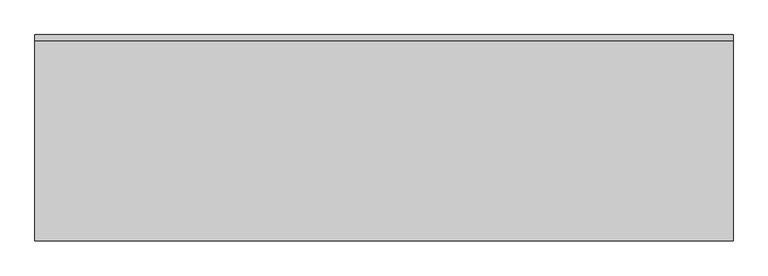
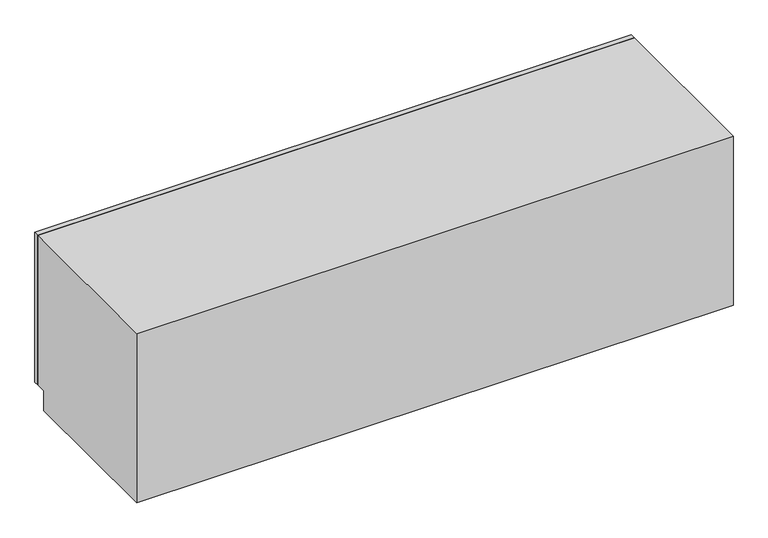
"""IFC4 building model written with IfcOpenShell, lengths in millimetres: furniture geometry, OD_CW_Base Cabinet : OD_CW_Base Cabinet."""

from ifc_helpers import new_model, si_unit, frame, origin, place, context, project, spatial, polyline, outline, extrude, source, transform, mapped, element, save


def furniture_ad26cfb4(model_context):
    return source(origin(), model_context, "Body", "SweptSolid", [
        extrude(outline(polyline([(18.7377049, 228.6), (18.7377049, 254.0), (2939.7377049, 254.0), (2939.7377049, 228.6), (18.7377049, 228.6)])), frame((0.0, 0.0, 101.6), z_axis=(0.0, 0.0, 1.0), x_axis=(1.0, 0.0, 0.0)), (0.0, 0.0, 1.0), 774.7),
        extrude(outline(polyline([(228.6, 876.3), (228.6, 101.6), (177.8, 101.6), (177.8, 0.0), (-609.6, 0.0), (-609.6, 876.3), (228.6, 876.3)])), frame((18.7377049, 0.0, 0.0), z_axis=(1.0, 0.0, 0.0), x_axis=(0.0, 1.0, 0.0)), (0.0, 0.0, 1.0), 2921.0),
    ])


if __name__ == "__main__":
    model = new_model("IFC4")
    model_context = context("Model", 3, world=origin())
    ifc_project = project(units=[si_unit("LENGTHUNIT", "METRE", prefix="MILLI")], contexts=[model_context])
    site = spatial("IfcSite", under=ifc_project)
    building = spatial("IfcBuilding", under=site)
    placement = place(None, origin())
    furniture_shape = furniture_ad26cfb4(model_context)
    element("IfcFurniture", 1, ObjectType="OD_CW_Base Cabinet : OD_CW_Base Cabinet", at=placement, inside=building, context=model_context, shape_type="MappedRepresentation", body=[
        mapped(furniture_shape, transform((0.0, 0.0, 0.0), x_axis=(1.0, 0.0, 0.0), y_axis=(0.0, 1.0, 0.0), z_axis=(0.0, 0.0, 1.0))),
    ])
    save(model, "model.ifc")

# Revit data of these elements
# Type "OD_CW_Base Cabinet : OD_CW_Base Cabinet"
#   OD_CW_Width [instance default] = 2' - 10"
#   OD_CW_Length [instance default] = 8' - 0"
#   OD_CW_Height [instance default] = 2' - 3"
#   Depth = 2' - 0"
#   Height = 3' - 0"
#   Width = 4' - 0"
#   OD_CW_Material_Front Panel [instance default] = none
#   OD_CW_Material_Body [instance default] = none
# Element 1 (IfcFurniture, "OD_CW_Base Cabinet : OD_CW_Base Cabinet")
#   OD_CW_Length = 9' - 7"
#   OD_CW_Height = 2' - 10 1/2"
#   Materials on its faces: "CASEWORK"
# Materials
#   "CASEWORK": class "Generic", colour RGB 181 181 181, transparency 0, Cost = 0
